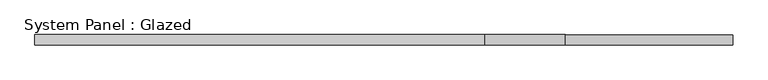
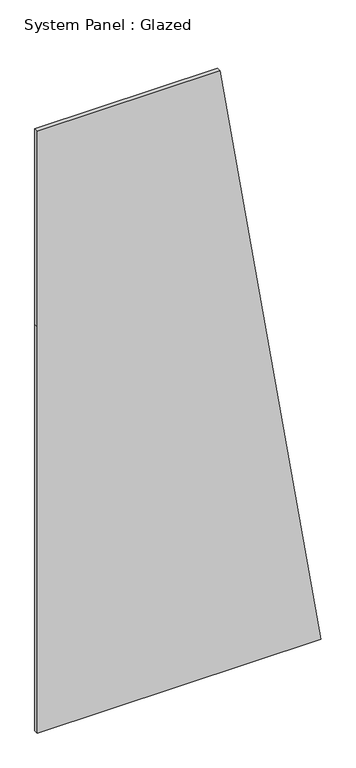
"""IFC4 building model written with IfcOpenShell, lengths in millimetres: plate geometry, System Panel : Glazed."""

from ifc_helpers import new_model, si_unit, frame, origin, place, context, project, spatial, polyline, outline, extrude, source, transform, mapped, element, save


def system_panel_glazed_1d752f2a(model_context):
    return source(origin(), model_context, "Body", "SweptSolid", [
        extrude(outline(polyline([(0.0, -681.1416347), (0.0, 681.1416347), (2052.1484522, 354.842633), (3050.0, 196.1806397), (3050.0, -681.1416347), (2060.0, -681.1416347), (0.0, -681.1416347)])), frame((0.0, 0.0, 0.0), z_axis=(0.0, 1.0, 0.0), x_axis=(0.0, 0.0, 1.0)), (0.0, 0.0, 1.0), 20.0),
    ])


if __name__ == "__main__":
    model = new_model("IFC4")
    model_context = context("Model", 3, world=origin())
    ifc_project = project(units=[si_unit("LENGTHUNIT", "METRE", prefix="MILLI")], contexts=[model_context])
    site = spatial("IfcSite", under=ifc_project)
    building = spatial("IfcBuilding", under=site)
    placement = place(None, origin())
    system_panel_glazed_shape = system_panel_glazed_1d752f2a(model_context)
    element("IfcPlate", 1, ObjectType="System Panel : Glazed", at=placement, inside=building, context=model_context, shape_type="MappedRepresentation", body=[
        mapped(system_panel_glazed_shape, transform((0.0, 0.0, 0.0), x_axis=(1.0, 0.0, 0.0), y_axis=(0.0, 1.0, 0.0), z_axis=(0.0, 0.0, 1.0))),
    ])
    save(model, "model.ifc")

# Revit data of these elements
# Type "System Panel : Glazed"
#   COBie.Type = no
# Element 1 (IfcPlate, "System Panel : Glazed")
#   Materials on its faces: "Glass"
# Materials
#   "Glass": class "Glass", colour RGB 0 128 192, transparency 0.75, Description = "Soda Lime Glass", Cost = 0
